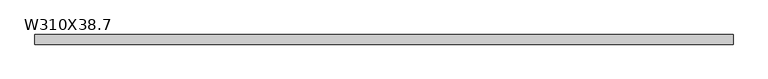
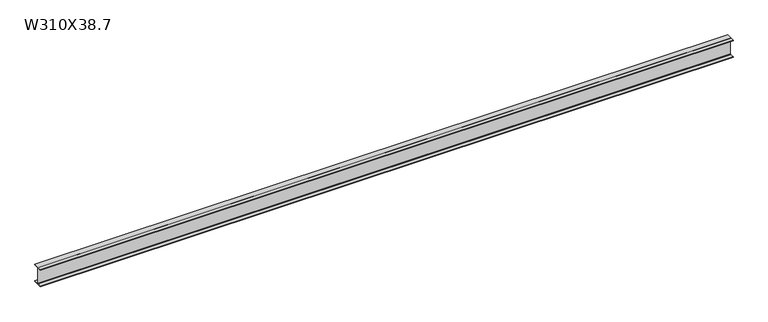
"""IFC4 building model written with IfcOpenShell, lengths in millimetres: beam geometry, M_W Shapes : W310X38.7."""

from ifc_helpers import new_model, si_unit, point, frame, frame_2d, origin, place, context, project, spatial, polyline, circle_curve, trimmed, segment, composite_curve, outline, extrude, source, transform, mapped, element, save


def w310x38_7_076b599a(model_context):
    return source(origin(), model_context, "Body", "SweptSolid", [
        extrude(outline(composite_curve([segment(polyline([(82.5, -145.35), (82.5, -155.0), (-82.5, -155.0), (-82.5, -145.35), (-10.57, -145.35)]), True, "CONTINUOUS"), segment(trimmed(circle_curve(frame_2d((-10.57, -137.7)), 7.65), [point((-10.57, -145.35))], [point((-2.92, -137.7))], True, "CARTESIAN"), True, "CONTINUOUS"), segment(polyline([(-2.92, -137.7), (-2.92, 137.7)]), True, "CONTINUOUS"), segment(trimmed(circle_curve(frame_2d((-10.57, 137.7)), 7.65), [point((-2.92, 137.7))], [point((-10.57, 145.35))], True, "CARTESIAN"), True, "CONTINUOUS"), segment(polyline([(-10.57, 145.35), (-82.5, 145.35), (-82.5, 155.0), (82.5, 155.0), (82.5, 145.35), (10.57, 145.35)]), True, "CONTINUOUS"), segment(trimmed(circle_curve(frame_2d((10.57, 137.7)), 7.65), [point((10.57, 145.35))], [point((2.92, 137.7))], True, "CARTESIAN"), True, "CONTINUOUS"), segment(polyline([(2.92, 137.7), (2.92, -137.7)]), True, "CONTINUOUS"), segment(trimmed(circle_curve(frame_2d((10.57, -137.7)), 7.65), [point((2.92, -137.7))], [point((10.57, -145.35))], True, "CARTESIAN"), True, "CONTINUOUS"), segment(polyline([(10.57, -145.35), (82.5, -145.35)]), True, "CONTINUOUS")], self_intersect=False)), frame((-6030.5, 0.0, 0.0), z_axis=(1.0, 0.0, 0.0), x_axis=(0.0, 1.0, 0.0)), (0.0, 0.0, 1.0), 11911.2),
    ])


if __name__ == "__main__":
    model = new_model("IFC4")
    model_context = context("Model", 3, world=origin())
    ifc_project = project(units=[si_unit("LENGTHUNIT", "METRE", prefix="MILLI")], contexts=[model_context])
    site = spatial("IfcSite", under=ifc_project)
    building = spatial("IfcBuilding", under=site)
    placement = place(None, origin())
    w310x38_7_shape = w310x38_7_076b599a(model_context)
    element("IfcBeam", 1, ObjectType="M_W Shapes : W310X38.7", at=placement, inside=building, context=model_context, shape_type="MappedRepresentation", body=[
        mapped(w310x38_7_shape, transform((0.0, 0.0, 0.0), x_axis=(1.0, 0.0, 0.0), y_axis=(0.0, 1.0, 0.0), z_axis=(0.0, 0.0, 1.0))),
    ])
    save(model, "model.ifc")

# Revit data of these elements
# Type "M_W Shapes : W310X38.7"
#   Section Name Key = "W12x26"
#   Width = 165 mm
#   Web Thickness = 5.84 mm
#   Web Fillet = 7.65 mm
#   Warping Constant = 163000 cm⁶
#   Torsional Moment of Inertia = 12.5 cm⁴
#   Section Area = 49.4 cm²
#   Plastic Modulus weak axis = 0.00473217 (stored number, unit not read)
#   Plastic Modulus strong axis = 0.0215419 (stored number, unit not read)
#   Perimeter = 1.25 m²/m
#   Nominal Weight = 379.516 N/m
#   Moment of Inertia weak axis = 720 cm⁴
#   Moment of Inertia strong axis = 8490 cm⁴
#   Height = 310 mm
#   Flange Thickness = 9.65 mm
#   Elastic Modulus weak axis = 0.00309003 (stored number, unit not read)
#   Elastic Modulus strong axis = 0.0193171 (stored number, unit not read)
#   Centroid Vertical = 155 mm
#   Centroid Horizontal = 82.5 mm
#   Length [instance default] = 1.5 m
#   Structural Material [instance default] = Steel, 45-345
#   Assembly Code = ""
# Element 1 (IfcBeam, "M_W Shapes : W310X38.7")
#   Materials on its faces: "Steel, 45-345"
# Materials
#   "Steel, 45-345": class "Metal", colour RGB 189 187 185, transparency 0, Description = "Steel 345 MPa", Cost = 0
